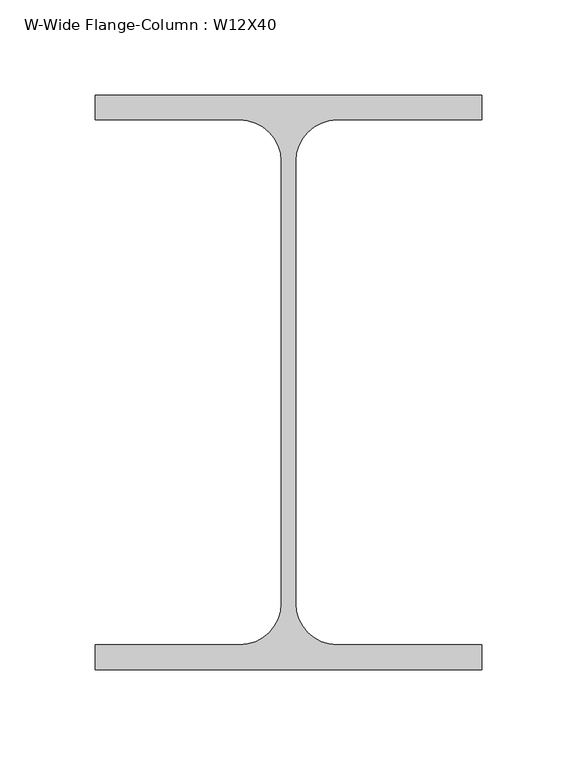
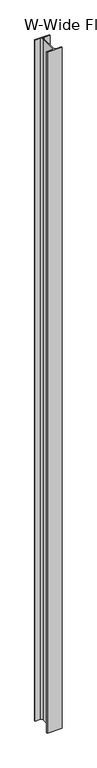
"""IFC4 building model written with IfcOpenShell, lengths in millimetres: column geometry, W-Wide Flange-Column : W12X40."""

from ifc_helpers import new_model, si_unit, point, frame, frame_2d, origin, place, context, project, spatial, polyline, circle_curve, trimmed, segment, composite_curve, outline, extrude, source, transform, mapped, element, save


def w_wide_flange_column_w12x40_d05c6117(model_context):
    return source(origin(), model_context, "Body", "SweptSolid", [
        extrude(outline(composite_curve([segment(polyline([(101.727, 151.13), (101.727, 138.049), (25.5905, 138.049)]), True, "CONTINUOUS"), segment(trimmed(circle_curve(frame_2d((25.5905, 116.205)), 21.844), [point((25.5905, 138.049))], [point((3.7465, 116.205))], True, "CARTESIAN"), True, "CONTINUOUS"), segment(polyline([(3.7465, 116.205), (3.7465, -116.205)]), True, "CONTINUOUS"), segment(trimmed(circle_curve(frame_2d((25.5905, -116.205)), 21.844), [point((3.7465, -116.205))], [point((25.5905, -138.049))], True, "CARTESIAN"), True, "CONTINUOUS"), segment(polyline([(25.5905, -138.049), (101.727, -138.049), (101.727, -151.13), (-101.727, -151.13), (-101.727, -138.049), (-25.5905, -138.049)]), True, "CONTINUOUS"), segment(trimmed(circle_curve(frame_2d((-25.5905, -116.205)), 21.844), [point((-25.5905, -138.049))], [point((-3.7465, -116.205))], True, "CARTESIAN"), True, "CONTINUOUS"), segment(polyline([(-3.7465, -116.205), (-3.7465, 116.205)]), True, "CONTINUOUS"), segment(trimmed(circle_curve(frame_2d((-25.5905, 116.205)), 21.844), [point((-3.7465, 116.205))], [point((-25.5905, 138.049))], True, "CARTESIAN"), True, "CONTINUOUS"), segment(polyline([(-25.5905, 138.049), (-101.727, 138.049), (-101.727, 151.13), (101.727, 151.13)]), True, "CONTINUOUS")], self_intersect=False)), frame((0.0, 0.0, 17627.6), z_axis=(0.0, 0.0, 1.0), x_axis=(1.0, 0.0, 0.0)), (0.0, 0.0, 1.0), 9956.8),
    ])


if __name__ == "__main__":
    model = new_model("IFC4")
    model_context = context("Model", 3, world=origin())
    ifc_project = project(units=[si_unit("LENGTHUNIT", "METRE", prefix="MILLI")], contexts=[model_context])
    site = spatial("IfcSite", under=ifc_project)
    building = spatial("IfcBuilding", under=site)
    placement = place(None, origin())
    w_wide_flange_column_w12x40_shape = w_wide_flange_column_w12x40_d05c6117(model_context)
    element("IfcColumn", 1, ObjectType="W-Wide Flange-Column : W12X40", at=placement, inside=building, context=model_context, shape_type="MappedRepresentation", body=[
        mapped(w_wide_flange_column_w12x40_shape, transform((0.0, 0.0, 0.0), x_axis=(1.0, 0.0, 0.0), y_axis=(0.0, 1.0, 0.0), z_axis=(0.0, 0.0, 1.0))),
    ])
    save(model, "model.ifc")

# Revit data of these elements
# Type "W-Wide Flange-Column : W12X40"
#   Assembly Code = "B10"
#   W = 40
#   bf = 0' - 8.01"
#   d = 0' - 11.9"
#   k = 0' - 1 3/8"
#   kr = 0' - 0.86"
#   tf = 0' - 0.515"
#   tw = 0' - 0.295"
#   A = 0.08125 SF
#   Structural Material [instance default] = Steel ASTM A992
# Element 1 (IfcColumn, "W-Wide Flange-Column : W12X40")
#   Materials on its faces: "Steel ASTM A992"
# Materials
#   "Steel ASTM A992": class "Metal", colour RGB 199 199 199, transparency 0, Description = "Structural steel 50ksi", Cost = 0
